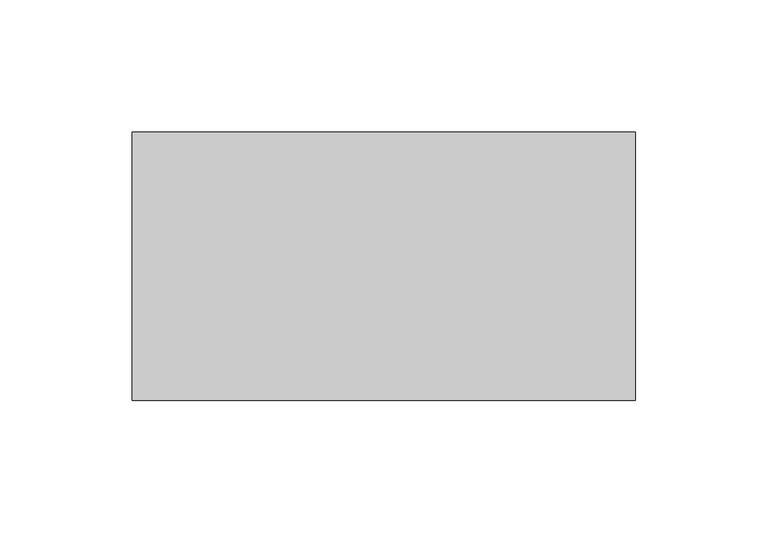
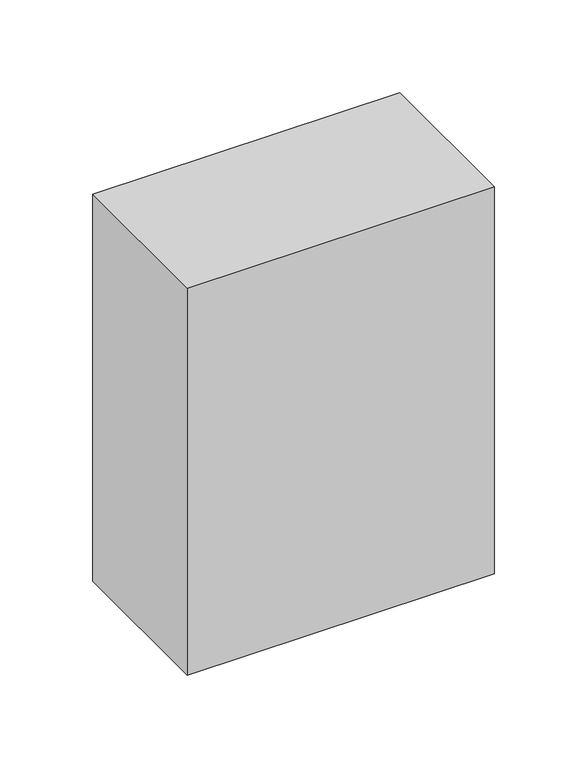
"""IFC4 building model written with IfcOpenShell, lengths in millimetres: proxy geometry, Seqm-Sanitary Napkin Disp-UH-3D : Seqm-Sanitary Napkin Disp-UH-3D."""

from ifc_helpers import new_model, si_unit, frame, origin, place, context, project, spatial, polyline, outline, extrude, source, transform, mapped, element, save


def specialty_equipment_d616f49c(model_context):
    return source(origin(), model_context, "Body", "SweptSolid", [
        extrude(outline(polyline([(95.25, 0.0), (95.25, -101.6), (-95.25, -101.6), (-95.25, 0.0), (95.25, 0.0)])), frame((0.0, 0.0, 482.6), z_axis=(0.0, 0.0, 1.0), x_axis=(1.0, 0.0, 0.0)), (0.0, 0.0, 1.0), 254.0),
    ])


if __name__ == "__main__":
    model = new_model("IFC4")
    model_context = context("Model", 3, world=origin())
    ifc_project = project(units=[si_unit("LENGTHUNIT", "METRE", prefix="MILLI")], contexts=[model_context])
    site = spatial("IfcSite", under=ifc_project)
    building = spatial("IfcBuilding", under=site)
    placement = place(None, origin())
    specialty_equipment_shape = specialty_equipment_d616f49c(model_context)
    element("IfcBuildingElementProxy", 1, Name="Seqm-Sanitary Napkin Disp-UH-3D : Seqm-Sanitary Napkin Disp-UH-3D", ObjectType="Seqm-Sanitary Napkin Disp-UH-3D : Seqm-Sanitary Napkin Disp-UH-3D", at=placement, inside=building, context=model_context, shape_type="MappedRepresentation", body=[
        mapped(specialty_equipment_shape, transform((0.0, 0.0, 0.0), x_axis=(1.0, 0.0, 0.0), y_axis=(0.0, 1.0, 0.0), z_axis=(0.0, 0.0, 1.0))),
    ])
    save(model, "model.ifc")

# Revit data of these elements
# Type "Seqm-Sanitary Napkin Disp-UH-3D : Seqm-Sanitary Napkin Disp-UH-3D"
#   Width = 0' - 7 1/2"
#   Height from Floor = 1' - 7"
#   Height = 0' - 10"
#   Depth = 0' - 4"
# Element 1 (IfcBuildingElementProxy, "Seqm-Sanitary Napkin Disp-UH-3D : Seqm-Sanitary Napkin Disp-UH-3D")
#   Materials on its faces: "NAPKIN DIPENSER (IF WOMEN'S)"
# Materials
#   "NAPKIN DIPENSER (IF WOMEN'S)": class "Generic", colour RGB 120 120 120, transparency 0, Cost = 0
